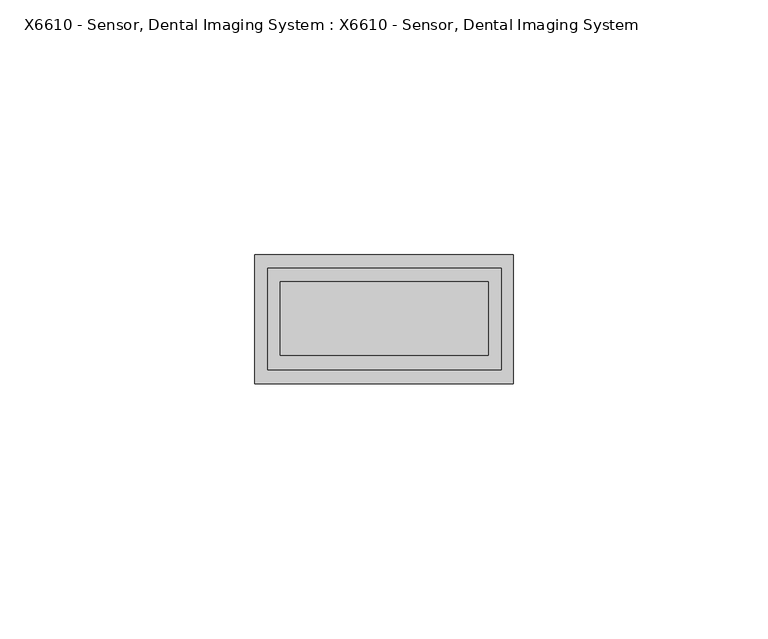
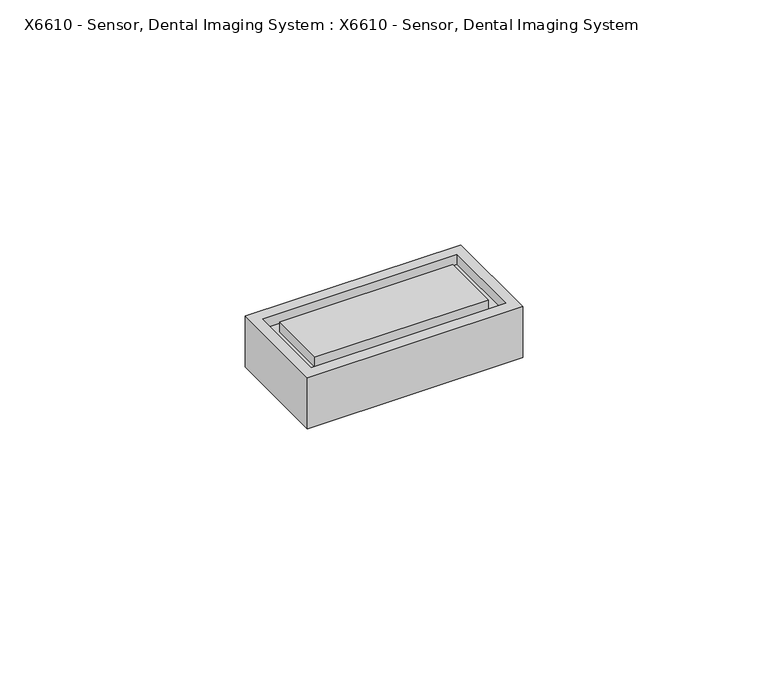
"""IFC4 building model written with IfcOpenShell, lengths in millimetres: proxy geometry, X6610 - Sensor, Dental Imaging System : X6610 - Sensor, Dental Imaging System."""

from ifc_helpers import new_model, si_unit, frame, origin, place, context, project, spatial, polyline, outline, extrude, faceted_brep, source, transform, mapped, element, save


def x6610_sensor_dental_imaging_system_x6610_sensor_dental_5278fb40(model_context):
    return source(origin(), model_context, "Body", "SolidModel", [
        extrude(outline(polyline([(20.4811453, -7.060747), (-20.3347495, -7.060747), (-20.3347495, 7.3741427), (20.4811453, 7.3741427), (20.4811453, -7.060747)])), frame((0.0, 0.0, 10.2472794), z_axis=(0.0, 0.0, 1.0), x_axis=(1.0, 0.0, 0.0)), (0.0, 0.0, 1.0), 2.4527206),
        faceted_brep([(25.4, 12.7, 12.7), (25.4, 12.7, 0.0), (-25.4, 12.7, 0.0), (-25.4, 12.7, 12.7), (25.4, -12.7, 12.7), (-25.4, -12.7, 12.7), (-25.4, -12.7, 0.0), (25.4, -12.7, 0.0), (-22.8050147, -9.9039698, 12.7), (-22.8050147, 10.029614, 12.7), (22.9818235, 10.029614, 12.7), (22.9818235, -9.9039698, 12.7), (25.4, 5.9907412, 2.9524929), (25.4, -6.0970829, 2.9524929), (25.4, -6.0970829, 7.2153756), (25.4, 5.9907412, 7.2153756), (22.9818235, -9.9039698, 10.2472794), (22.9818235, 10.029614, 10.2472794), (-22.8050147, 10.029614, 10.2472794), (-22.8050147, -9.9039698, 10.2472794), (17.7337242, 5.9907412, 7.2153756), (17.7337242, -6.0970829, 7.2153756), (17.7337242, -6.0970829, 2.9524929), (17.7337242, 5.9907412, 2.9524929)], [[[0, 1, 2, 3]], [[4, 5, 6, 7]], [[3, 5, 4, 0], [8, 9, 10, 11]], [[2, 6, 5, 3]], [[1, 7, 6, 2]], [[0, 4, 7, 1], [12, 13, 14, 15]], [[16, 17, 18, 19]], [[19, 8, 11, 16]], [[18, 9, 8, 19]], [[17, 10, 9, 18]], [[16, 11, 10, 17]], [[20, 21, 22, 23]], [[23, 12, 15, 20]], [[22, 13, 12, 23]], [[21, 14, 13, 22]], [[20, 15, 14, 21]]]),
        faceted_brep([(-25.4, -12.7, 12.7), (25.4, -12.7, 12.7), (25.4, 12.7, 12.7), (-25.4, 12.7, 12.7), (-25.4, 0.0, 12.7), (-22.8050147, -9.9039698, 12.7), (-22.8050147, 10.029614, 12.7), (22.9818235, 10.029614, 12.7), (22.9818235, -9.9039698, 12.7), (-25.4, -12.7, 0.0), (-25.4, 0.0, 0.0), (-25.4, 12.7, 0.0), (25.4, 12.7, 0.0), (25.4, -12.7, 0.0), (25.4, 5.9907412, 2.9524929), (25.4, -6.0970829, 2.9524929), (25.4, -6.0970829, 7.2153756), (25.4, 5.9907412, 7.2153756), (22.9818235, -9.9039698, 10.2472794), (22.9818235, 10.029614, 10.2472794), (-22.8050147, 10.029614, 10.2472794), (-22.8050147, -9.9039698, 10.2472794), (17.7337242, 5.9907412, 7.2153756), (17.7337242, -6.0970829, 7.2153756), (17.7337242, -6.0970829, 2.9524929), (17.7337242, 5.9907412, 2.9524929)], [[[0, 1, 2, 3, 4], [5, 6, 7, 8]], [[9, 10, 11, 12, 13]], [[4, 10, 9, 0]], [[3, 11, 10, 4]], [[2, 12, 11, 3]], [[1, 13, 12, 2], [14, 15, 16, 17]], [[0, 9, 13, 1]], [[18, 19, 20, 21]], [[21, 5, 8, 18]], [[20, 6, 5, 21]], [[19, 7, 6, 20]], [[18, 8, 7, 19]], [[22, 23, 24, 25]], [[25, 14, 17, 22]], [[24, 15, 14, 25]], [[23, 16, 15, 24]], [[22, 17, 16, 23]]]),
    ])


if __name__ == "__main__":
    model = new_model("IFC4")
    model_context = context("Model", 3, world=origin())
    ifc_project = project(units=[si_unit("LENGTHUNIT", "METRE", prefix="MILLI")], contexts=[model_context])
    site = spatial("IfcSite", under=ifc_project)
    building = spatial("IfcBuilding", under=site)
    placement = place(None, origin())
    x6610_sensor_dental_imaging_system_x6610_sensor_dental_shape = x6610_sensor_dental_imaging_system_x6610_sensor_dental_5278fb40(model_context)
    element("IfcBuildingElementProxy", 1, Name="X6610 - Sensor, Dental Imaging System : X6610 - Sensor, Dental Imaging System", ObjectType="X6610 - Sensor, Dental Imaging System : X6610 - Sensor, Dental Imaging System", at=placement, inside=building, context=model_context, shape_type="MappedRepresentation", body=[
        mapped(x6610_sensor_dental_imaging_system_x6610_sensor_dental_shape, transform((0.0, 0.0, 0.0), x_axis=(1.0, 0.0, 0.0), y_axis=(0.0, 1.0, 0.0), z_axis=(0.0, 0.0, 1.0))),
    ])
    save(model, "model.ifc")

# Revit data of these elements
# Type "X6610 - Sensor, Dental Imaging System : X6610 - Sensor, Dental Imaging System"
#   Watts2 = "0"
#   Watts1 = "0"
#   Unit_Issue = "EA"
#   UTIL_6_Misc = "-"
#   UTIL_5_NonMedGas = "-"
#   UTIL_4_MiscGas = "-"
#   UTIL_3_MedGas = "-"
#   UTIL_2_Elec = "-"
#   UTIL_1_WaterDrain = "-"
#   Nomenclature = "Sensor, Dental Imaging System"
#   NSN = ""
#   Location [instance default] = ""
#   JSN = "X6610"
#   Fund_Source_VA = "-"
#   Fund_Source_Navy = "-"
#   Fund_Source_Army = "-"
#   Fund_Source_AF = "-"
#   ELEC_Volts2 = "0"
#   ELEC_Volts1 = "0"
#   ELEC_Phase2 = "0"
#   ELEC_Phase1 = "0"
#   ELEC_HertzSwitch = "0"
#   ELEC_HertzDependent = "0"
#   ELEC_Hertz = "0"
#   ELEC_Amps2 = "0"
#   ELEC_Amps1 = "0"
#   DetailDescription = "A filmless digital imaging system using a sensor to acquire and digitize dental x-ray images for viewing, storing or printing. The sensor is used in conjunction with a film based x-ray system. Images are digitized and transmitted to a computer via a standard USB port and is compatible with laptop or desktop systems."
#   CAT_VA = "C"
#   CAT_Navy = "C"
#   CAT_IHS = "-"
#   CAT_Army = "C"
#   CAT_AF = "C"
#   BTUperhour = "0"
#   Weight_IP = 3
#   DIM_Width_IP = 0' - 2"
#   DIM_Height_IP = 0' - 0 1/2"
#   DIM_Depth_IP = 0' - 1"
# Element 1 (IfcBuildingElementProxy, "X6610 - Sensor, Dental Imaging System : X6610 - Sensor, Dental Imaging System")
#   Materials on its faces: "EquipSpace"
# Materials
#   "EquipSpace": class "Unassigned", colour RGB 221 217 195, transparency 0.5
